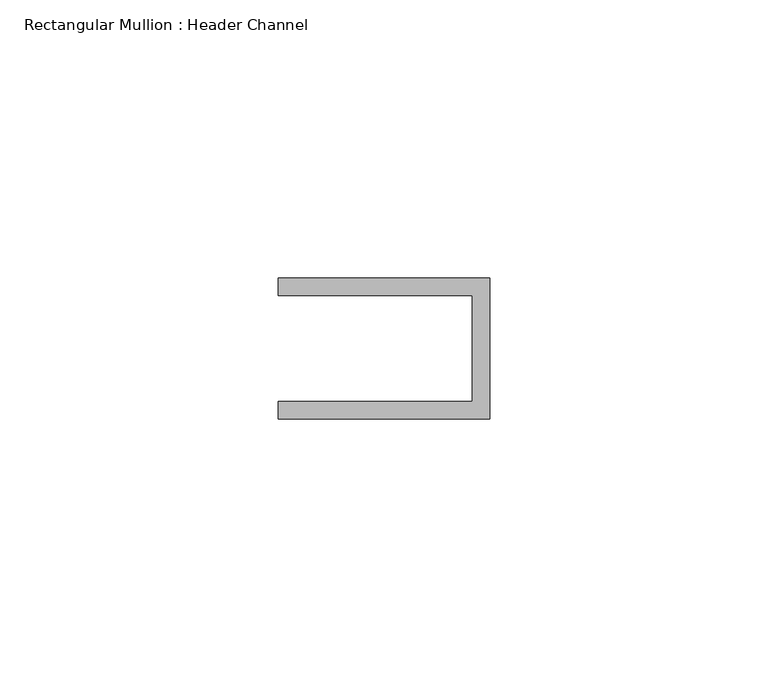
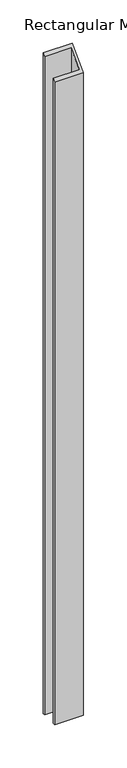
"""IFC4 building model written with IfcOpenShell, lengths in millimetres: member geometry, Rectangular Mullion : Header Channel."""

from ifc_helpers import new_model, si_unit, origin, place, context, project, spatial, faceted_brep, source, transform, mapped, element, save


def rectangular_mullion_header_channel_66cbb038(model_context):
    return source(origin(), model_context, "Body", "Brep", [
        faceted_brep([(0.0, -12.7, -914.4000002), (-38.1, -12.7, -914.4000002), (-38.1, -9.525, -914.4000002), (-3.175, -9.525, -914.4000002), (-3.175, 9.525, -914.4000002), (-38.1, 9.525, -914.4000002), (-38.1, 12.7, -914.4000002), (0.0, 12.7, -914.4000002), (0.0, 12.7, 12.7), (0.0, -12.7, -12.7), (-38.1, 12.7, 12.7), (-38.1, 9.525, 9.525), (-3.175, 9.525, 9.525), (-3.175, -9.525, -9.525), (-38.1, -9.525, -9.525), (-38.1, -12.7, -12.7)], [[[0, 1, 2, 3, 4, 5, 6, 7]], [[8, 9, 0, 7]], [[10, 8, 7, 6]], [[11, 10, 6, 5]], [[12, 11, 5, 4]], [[13, 12, 4, 3]], [[14, 13, 3, 2]], [[15, 14, 2, 1]], [[9, 15, 1, 0]], [[9, 8, 10, 11, 12, 13, 14, 15]]]),
    ])


if __name__ == "__main__":
    model = new_model("IFC4")
    model_context = context("Model", 3, world=origin())
    ifc_project = project(units=[si_unit("LENGTHUNIT", "METRE", prefix="MILLI")], contexts=[model_context])
    site = spatial("IfcSite", under=ifc_project)
    building = spatial("IfcBuilding", under=site)
    placement = place(None, origin())
    rectangular_mullion_header_channel_shape = rectangular_mullion_header_channel_66cbb038(model_context)
    element("IfcMember", 1, ObjectType="Rectangular Mullion : Header Channel", at=placement, inside=building, context=model_context, shape_type="MappedRepresentation", body=[
        mapped(rectangular_mullion_header_channel_shape, transform((0.0, 0.0, 0.0), x_axis=(1.0, 0.0, 0.0), y_axis=(0.0, 1.0, 0.0), z_axis=(0.0, 0.0, 1.0))),
    ])
    save(model, "model.ifc")

# Revit data of these elements
# Type "Rectangular Mullion : Header Channel"
#   built-in parameter 1007322 = 0.0833333 (stored number, unit not read)
#   built-in parameter 1007321 = -0.03125 (stored number, unit not read)
#   built-in parameter 1007320 = 0.0416667 (stored number, unit not read)
# Element 1 (IfcMember, "Rectangular Mullion : Header Channel")
#   Materials on its faces: "ALUM"
# Materials
#   "ALUM": class "Generic", colour RGB 157 157 157, transparency 0, Cost = 0
